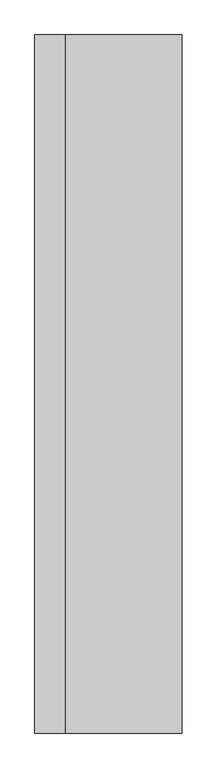
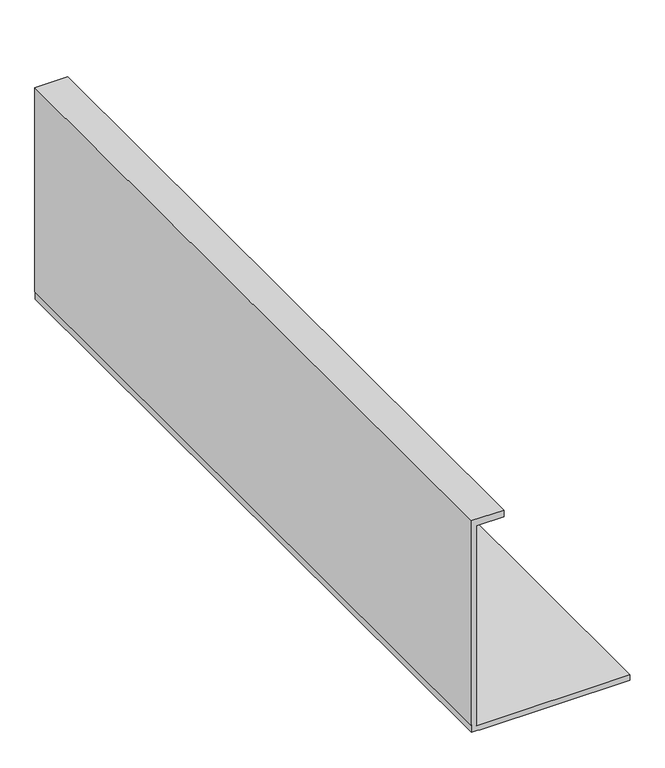
"""IFC4 building model written with IfcOpenShell, lengths in millimetres: proxy geometry, Gypsum023 8100 : Gypsum023 8100."""

from ifc_helpers import new_model, si_unit, frame, origin, place, context, project, spatial, polyline, outline, extrude, source, transform, mapped, element, save


def generic_models_519f700a(model_context):
    return source(origin(), model_context, "Body", "SweptSolid", [
        extrude(outline(polyline([(39557.071, 7625.6892957), (39572.946, 7625.6892957), (39572.946, 7218.5762049), (40131.746, 7218.5762049), (40131.746, 7290.9824219), (40150.796, 7290.9824219), (40150.796, 7203.5713569), (39579.5041839, 7203.5713569), (39579.5041839, 7204.8513569), (39558.351, 7204.8513569), (39558.351, 7226.0045408), (39557.071, 7226.0045408), (39557.071, 7625.6892957)])), frame((0.0, -3747.9491938, 0.0), z_axis=(0.0, 1.0, 0.0), x_axis=(0.0, 0.0, 1.0)), (0.0, 0.0, 1.0), 1999.85),
    ])


if __name__ == "__main__":
    model = new_model("IFC4")
    model_context = context("Model", 3, world=origin())
    ifc_project = project(units=[si_unit("LENGTHUNIT", "METRE", prefix="MILLI")], contexts=[model_context])
    site = spatial("IfcSite", under=ifc_project)
    building = spatial("IfcBuilding", under=site)
    placement = place(None, origin())
    generic_models_shape = generic_models_519f700a(model_context)
    element("IfcBuildingElementProxy", 1, Name="Gypsum023 8100 : Gypsum023 8100", ObjectType="Gypsum023 8100 : Gypsum023 8100", at=placement, inside=building, context=model_context, shape_type="MappedRepresentation", body=[
        mapped(generic_models_shape, transform((0.0, 0.0, 0.0), x_axis=(1.0, 0.0, 0.0), y_axis=(0.0, 1.0, 0.0), z_axis=(0.0, 0.0, 1.0))),
    ])
    save(model, "model.ifc")

# Revit data of these elements
# Type "Gypsum023 8100 : Gypsum023 8100"
#   NameOverride = "Gypsum023"
# Element 1 (IfcBuildingElementProxy, "Gypsum023 8100 : Gypsum023 8100")
#   Materials on its faces: "5/8\" GYPSUM BOARD"
# Materials
#   "5/8\" GYPSUM BOARD": class "Unassigned", colour RGB 255 255 255, transparency 0, Cost = 0
